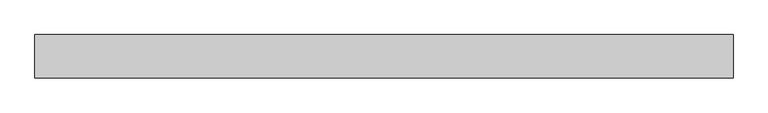
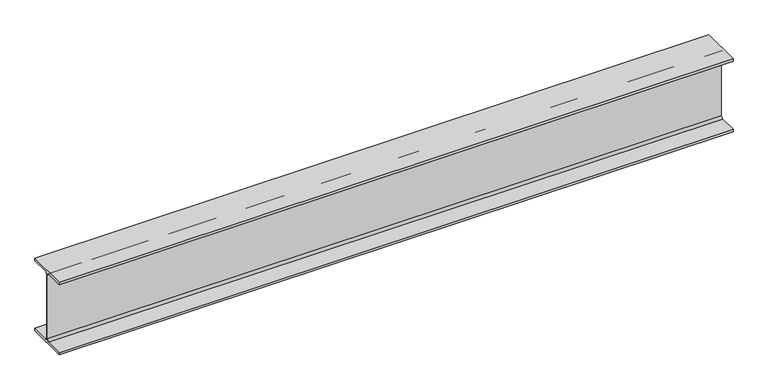
"""IFC4 building model written with IfcOpenShell, lengths in millimetres: beam geometry, Old_Steel Beam_H-KSD3502 : H_SB_ASB_H-194×150x6x9."""

from ifc_helpers import new_model, si_unit, point, frame, frame_2d, origin, place, context, project, spatial, polyline, circle_curve, trimmed, segment, composite_curve, outline, extrude, source, transform, mapped, element, save


def beam_c6f56534(model_context):
    return source(origin(), model_context, "Body", "SweptSolid", [
        extrude(outline(composite_curve([segment(polyline([(-82.5, -141.5), (-11.9, -141.5)]), True, "CONTINUOUS"), segment(trimmed(circle_curve(frame_2d((-11.9, -132.6)), 8.9), [point((-11.9, -141.5))], [point((-3.0, -132.6))], True, "CARTESIAN"), True, "CONTINUOUS"), segment(polyline([(-3.0, -132.6), (-3.0, 132.6)]), True, "CONTINUOUS"), segment(trimmed(circle_curve(frame_2d((-11.9, 132.6)), 8.9), [point((-3.0, 132.6))], [point((-11.9, 141.5))], True, "CARTESIAN"), True, "CONTINUOUS"), segment(polyline([(-11.9, 141.5), (-82.5, 141.5), (-82.5, 151.7), (82.5, 151.7), (82.5, 141.5), (11.9, 141.5)]), True, "CONTINUOUS"), segment(trimmed(circle_curve(frame_2d((11.9, 132.6)), 8.9), [point((11.9, 141.5))], [point((3.0, 132.6))], True, "CARTESIAN"), True, "CONTINUOUS"), segment(polyline([(3.0, 132.6), (3.0, -132.6)]), True, "CONTINUOUS"), segment(trimmed(circle_curve(frame_2d((11.9, -132.6)), 8.9), [point((3.0, -132.6))], [point((11.9, -141.5))], True, "CARTESIAN"), True, "CONTINUOUS"), segment(polyline([(11.9, -141.5), (82.5, -141.5), (82.5, -151.7), (-82.5, -151.7), (-82.5, -141.5)]), True, "CONTINUOUS")], self_intersect=False)), frame((-1106.6961534, 0.0, 0.0), z_axis=(1.0, 0.0, 0.0), x_axis=(0.0, 1.0, 0.0)), (0.0, 0.0, 1.0), 2655.7235444),
    ])


if __name__ == "__main__":
    model = new_model("IFC4")
    model_context = context("Model", 3, world=origin())
    ifc_project = project(units=[si_unit("LENGTHUNIT", "METRE", prefix="MILLI")], contexts=[model_context])
    site = spatial("IfcSite", under=ifc_project)
    building = spatial("IfcBuilding", under=site)
    placement = place(None, origin())
    beam_shape = beam_c6f56534(model_context)
    element("IfcBeam", 1, ObjectType="Old_Steel Beam_H-KSD3502 : H_SB_ASB_H-194×150x6x9", at=placement, inside=building, context=model_context, shape_type="MappedRepresentation", body=[
        mapped(beam_shape, transform((0.0, 0.0, 0.0), x_axis=(1.0, 0.0, 0.0), y_axis=(0.0, 1.0, 0.0), z_axis=(0.0, 0.0, 1.0))),
    ])
    save(model, "model.ifc")

# Revit data of these elements
# Type "Old_Steel Beam_H-KSD3502 : H_SB_ASB_H-194×150x6x9"
#   Width = 15.0 cm
#   Web Thickness = 0.6 cm
#   Web Fillet = 1.3 cm
#   Warping Constant = 43316.0 cm⁶
#   Torsional Moment of Inertia = 8.622 cm⁴
#   Torsional Modulus = 1.0 cm³
#   Section Area = 39.01 cm²
#   Plastic Modulus weak axis = 104.0 cm³
#   Plastic Modulus strong axis = 309.0 cm³
#   Perimeter = 0.95 m²/m
#   Nominal Weight = 30.60 kgf/m
#   Moment of Inertia weak axis = 507.00 cm⁴
#   Moment of Inertia strong axis = 2690.00 cm⁴
#   Height = 19.4 cm
#   Flange Thickness = 0.9 cm
#   Elastic Modulus weak axis = 67.6 cm³
#   Elastic Modulus strong axis = 277.0 cm³
#   Centroid Vertical = 9.7 cm
#   Centroid Horizontal = 7.5 cm
#   Length [instance default] = 1.5240 m
#   Structural Material [instance default] = Steel, 45-345
#   Assembly Code = ""
# Element 1 (IfcBeam, "Old_Steel Beam_H-KSD3502 : H_SB_ASB_H-194×150x6x9")
#   Structural Material = none
# Materials
#   "Steel, 45-345": class "Metal", colour RGB 189 187 185, transparency 0, Description = "Steel 345 MPa", Cost = 0
